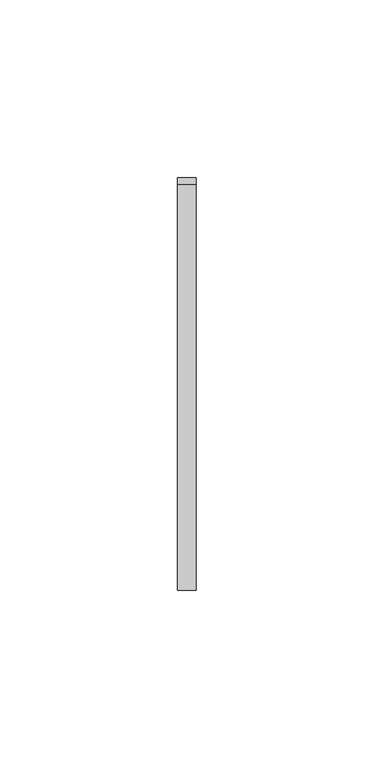
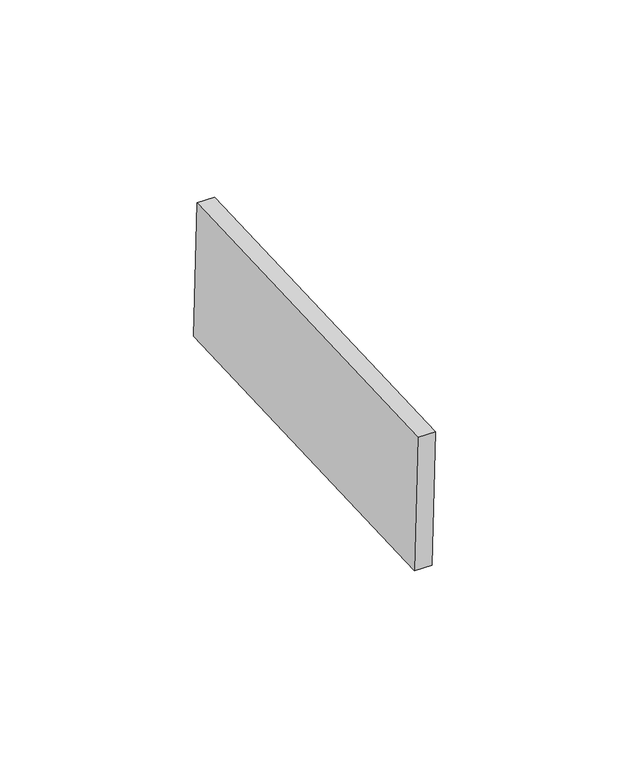
"""IFC4 building model written with IfcOpenShell, lengths in millimetres: proxy geometry, Inner panel:Inner panel:1:Inner panel:1 : Inner panel:Inner panel:300324:2:Inner panel:1:Inner panel:1 : Inner panel:Inner panel:300324:2 : Inner panel:Inner panel:1:Inner panel:1 : Inner panel:Inner panel:300324:300043:55 : Inner panel:Inner panel:1:Inner panel:1 : Inner panel:Inner panel:300324:2:Inner panel:1:Inner panel:1 : Inner panel:Inner panel:300324:2 : Inner panel:Inner panel:1:Inner panel:1 : Inner panel:Inner panel:300324:300043:308120."""

from ifc_helpers import new_model, si_unit, frame, origin, place, context, project, spatial, polyline, outline, extrude, source, transform, mapped, element, save


def generic_models_5b4f5c44(model_context):
    return source(origin(), model_context, "Body", "SweptSolid", [
        extrude(outline(polyline([(0.0, -114.2999999), (0.0, 0.0), (5.2138089, 0.0), (5.2138089, -114.2999999), (0.0, -114.2999999)])), frame((591904.595117, -566950.1308393, 8857.6957503), z_axis=(0.0, -0.04163054471215927, 0.9991330730923529), x_axis=(-1.0, 0.0, 0.0)), (0.0, 0.0, 1.0), 43.2233908),
    ])


if __name__ == "__main__":
    model = new_model("IFC4")
    model_context = context("Model", 3, world=origin())
    ifc_project = project(units=[si_unit("LENGTHUNIT", "METRE", prefix="MILLI")], contexts=[model_context])
    site = spatial("IfcSite", under=ifc_project)
    building = spatial("IfcBuilding", under=site)
    placement = place(None, origin())
    generic_models_shape = generic_models_5b4f5c44(model_context)
    element("IfcBuildingElementProxy", 1, Name="Inner panel:Inner panel:1:Inner panel:1 : Inner panel:Inner panel:300324:2:Inner panel:1:Inner panel:1 : Inner panel:Inner panel:300324:2 : Inner panel:Inner panel:1:Inner panel:1 : Inner panel:Inner panel:300324:300043:55 : Inner panel:Inner panel:1:Inner panel:1 : Inner panel:Inner panel:300324:2:Inner panel:1:Inner panel:1 : Inner panel:Inner panel:300324:2 : Inner panel:Inner panel:1:Inner panel:1 : Inner panel:Inner panel:300324:300043:308120", ObjectType="Inner panel:Inner panel:1:Inner panel:1 : Inner panel:Inner panel:300324:2:Inner panel:1:Inner panel:1 : Inner panel:Inner panel:300324:2 : Inner panel:Inner panel:1:Inner panel:1 : Inner panel:Inner panel:300324:300043:55 : Inner panel:Inner panel:1:Inner panel:1 : Inner panel:Inner panel:300324:2:Inner panel:1:Inner panel:1 : Inner panel:Inner panel:300324:2 : Inner panel:Inner panel:1:Inner panel:1 : Inner panel:Inner panel:300324:300043:308120", at=placement, inside=building, context=model_context, shape_type="MappedRepresentation", body=[
        mapped(generic_models_shape, transform((0.0, 0.0, 0.0), x_axis=(1.0, 0.0, 0.0), y_axis=(0.0, 1.0, 0.0), z_axis=(0.0, 0.0, 1.0))),
    ])
    save(model, "model.ifc")

# Revit data of these elements
# Type "Inner panel:Inner panel:1:Inner panel:1 : Inner panel:Inner panel:300324:2:Inner panel:1:Inner panel:1 : Inner panel:Inner panel:300324:2 : Inner panel:Inner panel:1:Inner panel:1 : Inner panel:Inner panel:300324:300043:55 : Inner panel:Inner panel:1:Inner panel:1 : Inner panel:Inner panel:300324:2:Inner panel:1:Inner panel:1 : Inner panel:Inner panel:300324:2 : Inner panel:Inner panel:1:Inner panel:1 : Inner panel:Inner panel:300324:300043:308120"
#   NameOverride = "Inner panel:Inner panel:1:Inner panel:1 : Inner panel:Inner panel:300324:2:Inner panel:1:Inner panel:1 : Inner panel:Inner panel:300324:2 : Inner panel:Inner panel:1:Inner panel:1 : Inner panel:Inner panel:300324:300043:308120"
#   ObjectTypeOverride = "Inner panel:1:Inner panel:1 : Inner panel:Inner panel:300324:2 : Inner panel:Inner panel:1:Inner panel:1 : Inner panel:Inner panel:300324:300043"
#   Reference = "Inner panel"
#   Tag = "308120"
# Element 1 (IfcBuildingElementProxy, "Inner panel:Inner panel:1:Inner panel:1 : Inner panel:Inner panel:300324:2:Inner panel:1:Inner panel:1 : Inner panel:Inner panel:300324:2 : Inner panel:Inner panel:1:Inner panel:1 : Inner panel:Inner panel:300324:300043:55 : Inner panel:Inner panel:1:Inner panel:1 : Inner panel:Inner panel:300324:2:Inner panel:1:Inner panel:1 : Inner panel:Inner panel:300324:2 : Inner panel:Inner panel:1:Inner panel:1 : Inner panel:Inner panel:300324:300043:308120")
#   Materials on its faces: "SLIDING CLIP"
# Materials
#   "SLIDING CLIP": class "Generic", colour RGB 120 120 120, transparency 0, Cost = 0
